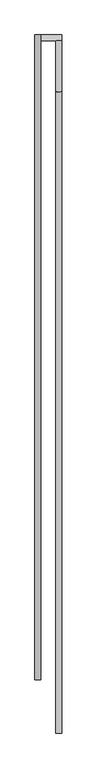
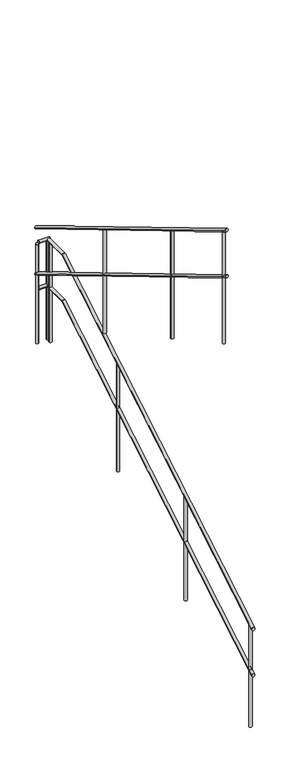
"""IFC4 building model written with IfcOpenShell, lengths in millimetres: railing geometry."""

from ifc_helpers import new_model, si_unit, point, frame, frame_2d, origin, place, context, project, spatial, circle_curve, ellipse_curve, trimmed, segment, composite_curve, outline, extrude, source, transform, mapped, element, save
from ifc_brep_helpers import plane_surface, cylinder_surface, advanced_brep


def railing_6fbbbaa8(model_context):
    return source(origin(), model_context, "Body", "SolidModel", [
        advanced_brep(
        [(11545.1052251, 14699.5208589, 749.8338893), (11515.1052251, 14699.5208589, 749.8338893), (11545.1052251, 18329.5208589, 2760.0), (11515.1052251, 18329.5208589, 2760.0), (11545.1052251, 18063.6609247, 2760.0), (11515.1052251, 18063.6609247, 2760.0)],
        [
            (0, 1, ellipse_curve(frame((11530.1052251, 14699.5208589, 749.8338893), z_axis=(0.0, -1.0, 0.0), x_axis=(0.0, 0.0, -1.0)), 17.4738031, 15.0)),
            (1, 0, ellipse_curve(frame((11530.1052251, 14699.5208589, 749.8338893), z_axis=(0.0, -1.0, 0.0), x_axis=(0.0, 0.0, -1.0)), 17.4738031, 15.0)),
            (2, 3, circle_curve(frame((11530.1052251, 18329.5208589, 2760.0), z_axis=(0.0, 1.0, 0.0), x_axis=(-1.0, 0.0, 0.0)), 15.0)),
            (3, 2, circle_curve(frame((11530.1052251, 18329.5208589, 2760.0), z_axis=(0.0, 1.0, 0.0), x_axis=(-1.0, 0.0, 0.0)), 15.0)),
            (0, 4),
            (4, 5, ellipse_curve(frame((11530.1052251, 18063.6609247, 2760.0), z_axis=(0.0, -0.9639574411334471, -0.26605648213012423), x_axis=(0.0, 0.2660564821301243, -0.9639574411334468)), 15.560853, 15.0)),
            (5, 1),
            (5, 4, ellipse_curve(frame((11530.1052251, 18063.6609247, 2760.0), z_axis=(0.0, -0.9639574411334471, -0.26605648213012423), x_axis=(0.0, 0.2660564821301243, -0.9639574411334468)), 15.560853, 15.0)),
            (4, 2),
            (3, 5),
        ],
        [
            plane_surface(frame((11530.1052251, 14699.5208589, 767.3076923), z_axis=(0.0, -1.0, 0.0), x_axis=(0.0, 0.0, 1.0))),
            plane_surface(frame((11530.1052251, 18329.5208589, 2775.0), z_axis=(0.0, 1.0, 0.0), x_axis=(0.0, 0.0, 1.0))),
            cylinder_surface(frame((11530.1052251, 14707.2148727, 754.4312739), z_axis=(0.0, -0.8584278966330859, -0.5129342514222422), x_axis=(-1.0, 0.0, 0.0)), 15.0),
            cylinder_surface(frame((11530.1052251, 18059.5208589, 2760.0), z_axis=(0.0, -1.0, 0.0), x_axis=(-1.0, 0.0, 0.0)), 15.0),
        ],
        [
            (0, [[1, 2]]),
            (1, [[3, 4]]),
            (2, [[-1, 5, 6, 7]]),
            (2, [[-2, -7, 8, -5]]),
            (3, [[-6, 9, -4, 10]]),
            (3, [[-8, -10, -3, -9]]),
        ],
    ),
        advanced_brep(
        [(11545.1052251, 18359.5208589, 2760.0), (11545.1052251, 18329.5208589, 2760.0), (11435.1052251, 18359.5208589, 2760.0), (11435.1052251, 18329.5208589, 2760.0)],
        [
            (0, 1, circle_curve(frame((11545.1052251, 18344.5208589, 2760.0), z_axis=(1.0, 0.0, 0.0), x_axis=(0.0, -1.0, 0.0)), 15.0)),
            (1, 0, circle_curve(frame((11545.1052251, 18344.5208589, 2760.0), z_axis=(1.0, 0.0, 0.0), x_axis=(0.0, -1.0, 0.0)), 15.0)),
            (2, 3, circle_curve(frame((11435.1052251, 18344.5208589, 2760.0), z_axis=(-1.0, 0.0, 0.0), x_axis=(0.0, -1.0, 0.0)), 15.0)),
            (3, 2, circle_curve(frame((11435.1052251, 18344.5208589, 2760.0), z_axis=(-1.0, 0.0, 0.0), x_axis=(0.0, -1.0, 0.0)), 15.0)),
            (0, 2),
            (3, 1),
        ],
        [
            plane_surface(frame((11545.1052251, 18344.5208589, 2775.0), z_axis=(1.0, 0.0, 0.0), x_axis=(0.0, -1.0, 0.0))),
            plane_surface(frame((11435.1052251, 18344.5208589, 2775.0), z_axis=(-1.0, 0.0, 0.0), x_axis=(0.0, -1.0, 0.0))),
            cylinder_surface(frame((11545.1052251, 18344.5208589, 2760.0), z_axis=(1.0, 0.0, 0.0), x_axis=(0.0, -1.0, 0.0)), 15.0),
        ],
        [
            (0, [[1, 2]]),
            (1, [[3, 4]]),
            (2, [[-1, 5, -4, 6]]),
            (2, [[-2, -6, -3, -5]]),
        ],
    ),
        advanced_brep(
        [(11405.1052251, 18359.5208589, 2912.8833398), (11435.1052251, 18359.5208589, 2912.8833398), (11405.1052251, 14979.5208589, 4932.5261969), (11435.1052251, 14979.5208589, 4932.5261969)],
        [
            (0, 1, ellipse_curve(frame((11420.1052251, 18359.5208589, 2912.8833398), z_axis=(0.0, 1.0, 0.0), x_axis=(0.0, 0.0, -1.0)), 17.4738031, 15.0)),
            (1, 0, ellipse_curve(frame((11420.1052251, 18359.5208589, 2912.8833398), z_axis=(0.0, 1.0, 0.0), x_axis=(0.0, 0.0, -1.0)), 17.4738031, 15.0)),
            (2, 3, ellipse_curve(frame((11420.1052251, 14979.5208589, 4932.5261969), z_axis=(0.0, -1.0, 0.0), x_axis=(0.0, 0.0, -1.0)), 17.4738031, 15.0)),
            (3, 2, ellipse_curve(frame((11420.1052251, 14979.5208589, 4932.5261969), z_axis=(0.0, -1.0, 0.0), x_axis=(0.0, 0.0, -1.0)), 17.4738031, 15.0)),
            (0, 2),
            (3, 1),
        ],
        [
            plane_surface(frame((11420.1052251, 18359.5208589, 2930.3571429), z_axis=(0.0, 1.0, 0.0), x_axis=(0.0, 0.0, -1.0))),
            plane_surface(frame((11420.1052251, 14979.5208589, 4950.0), z_axis=(0.0, -1.0, 0.0), x_axis=(0.0, 0.0, -1.0))),
            cylinder_surface(frame((11420.1052251, 18351.8268451, 2917.4807244), z_axis=(0.0, 0.8584278966330859, -0.5129342514222421), x_axis=(1.0, 0.0, 0.0)), 15.0),
        ],
        [
            (0, [[1, 2]]),
            (1, [[3, 4]]),
            (2, [[-1, 5, -4, 6]]),
            (2, [[-2, -6, -3, -5]]),
        ],
    ),
        advanced_brep(
        [(11545.1052251, 14699.5208589, 1249.8338893), (11515.1052251, 14699.5208589, 1249.8338893), (11545.1052251, 18063.6609247, 3260.0), (11515.1052251, 18063.6609247, 3260.0), (11545.1052251, 18329.5208589, 3260.0), (11515.1052251, 18329.5208589, 3260.0)],
        [
            (0, 1, ellipse_curve(frame((11530.1052251, 14699.5208589, 1249.8338893), z_axis=(0.0, -1.0, 0.0), x_axis=(0.0, 0.0, -1.0)), 17.4738031, 15.0)),
            (1, 0, ellipse_curve(frame((11530.1052251, 14699.5208589, 1249.8338893), z_axis=(0.0, -1.0, 0.0), x_axis=(0.0, 0.0, -1.0)), 17.4738031, 15.0)),
            (0, 2),
            (2, 3, ellipse_curve(frame((11530.1052251, 18063.6609247, 3260.0), z_axis=(0.0, -0.9639574411334471, -0.26605648213012423), x_axis=(0.0, 0.2660564821301243, -0.9639574411334468)), 15.560853, 15.0)),
            (3, 1),
            (3, 2, ellipse_curve(frame((11530.1052251, 18063.6609247, 3260.0), z_axis=(0.0, -0.9639574411334471, -0.26605648213012423), x_axis=(0.0, 0.2660564821301243, -0.9639574411334468)), 15.560853, 15.0)),
            (4, 5, circle_curve(frame((11530.1052251, 18329.5208589, 3260.0), z_axis=(0.0, 1.0, 0.0), x_axis=(-1.0, 0.0, 0.0)), 15.0)),
            (5, 4, circle_curve(frame((11530.1052251, 18329.5208589, 3260.0), z_axis=(0.0, 1.0, 0.0), x_axis=(-1.0, 0.0, 0.0)), 15.0)),
            (2, 4),
            (5, 3),
        ],
        [
            plane_surface(frame((11530.1052251, 14699.5208589, 1267.3076923), z_axis=(0.0, -1.0, 0.0), x_axis=(0.0, 0.0, 1.0))),
            cylinder_surface(frame((11530.1052251, 14707.2148727, 1254.4312739), z_axis=(0.0, -0.8584278966330859, -0.5129342514222422), x_axis=(-1.0, 0.0, 0.0)), 15.0),
            plane_surface(frame((11530.1052251, 18329.5208589, 3275.0), z_axis=(0.0, 1.0, 0.0), x_axis=(0.0, 0.0, 1.0))),
            cylinder_surface(frame((11530.1052251, 18059.5208589, 3260.0), z_axis=(0.0, -1.0, 0.0), x_axis=(-1.0, 0.0, 0.0)), 15.0),
        ],
        [
            (0, [[1, 2]]),
            (1, [[-1, 3, 4, 5]]),
            (1, [[-2, -5, 6, -3]]),
            (2, [[7, 8]]),
            (3, [[-4, 9, -8, 10]]),
            (3, [[-6, -10, -7, -9]]),
        ],
    ),
        advanced_brep(
        [(11545.1052251, 18359.5208589, 3260.0), (11545.1052251, 18329.5208589, 3260.0), (11435.1052251, 18359.5208589, 3260.0), (11435.1052251, 18329.5208589, 3260.0)],
        [
            (0, 1, circle_curve(frame((11545.1052251, 18344.5208589, 3260.0), z_axis=(1.0, 0.0, 0.0), x_axis=(0.0, -1.0, 0.0)), 15.0)),
            (1, 0, circle_curve(frame((11545.1052251, 18344.5208589, 3260.0), z_axis=(1.0, 0.0, 0.0), x_axis=(0.0, -1.0, 0.0)), 15.0)),
            (2, 3, circle_curve(frame((11435.1052251, 18344.5208589, 3260.0), z_axis=(-1.0, 0.0, 0.0), x_axis=(0.0, -1.0, 0.0)), 15.0)),
            (3, 2, circle_curve(frame((11435.1052251, 18344.5208589, 3260.0), z_axis=(-1.0, 0.0, 0.0), x_axis=(0.0, -1.0, 0.0)), 15.0)),
            (0, 2),
            (3, 1),
        ],
        [
            plane_surface(frame((11545.1052251, 18344.5208589, 3275.0), z_axis=(1.0, 0.0, 0.0), x_axis=(0.0, -1.0, 0.0))),
            plane_surface(frame((11435.1052251, 18344.5208589, 3275.0), z_axis=(-1.0, 0.0, 0.0), x_axis=(0.0, -1.0, 0.0))),
            cylinder_surface(frame((11545.1052251, 18344.5208589, 3260.0), z_axis=(1.0, 0.0, 0.0), x_axis=(0.0, -1.0, 0.0)), 15.0),
        ],
        [
            (0, [[1, 2]]),
            (1, [[3, 4]]),
            (2, [[-1, 5, -4, 6]]),
            (2, [[-2, -6, -3, -5]]),
        ],
    ),
        advanced_brep(
        [(11405.1052251, 18359.5208589, 3412.8833398), (11435.1052251, 18359.5208589, 3412.8833398), (11405.1052251, 14979.5208589, 5432.5261969), (11435.1052251, 14979.5208589, 5432.5261969)],
        [
            (0, 1, ellipse_curve(frame((11420.1052251, 18359.5208589, 3412.8833398), z_axis=(0.0, 1.0, 0.0), x_axis=(0.0, 0.0, -1.0)), 17.4738031, 15.0)),
            (1, 0, ellipse_curve(frame((11420.1052251, 18359.5208589, 3412.8833398), z_axis=(0.0, 1.0, 0.0), x_axis=(0.0, 0.0, -1.0)), 17.4738031, 15.0)),
            (2, 3, ellipse_curve(frame((11420.1052251, 14979.5208589, 5432.5261969), z_axis=(0.0, -1.0, 0.0), x_axis=(0.0, 0.0, -1.0)), 17.4738031, 15.0)),
            (3, 2, ellipse_curve(frame((11420.1052251, 14979.5208589, 5432.5261969), z_axis=(0.0, -1.0, 0.0), x_axis=(0.0, 0.0, -1.0)), 17.4738031, 15.0)),
            (0, 2),
            (3, 1),
        ],
        [
            plane_surface(frame((11420.1052251, 18359.5208589, 3430.3571429), z_axis=(0.0, 1.0, 0.0), x_axis=(0.0, 0.0, -1.0))),
            plane_surface(frame((11420.1052251, 14979.5208589, 5450.0), z_axis=(0.0, -1.0, 0.0), x_axis=(0.0, 0.0, -1.0))),
            cylinder_surface(frame((11420.1052251, 18351.8268451, 3417.4807244), z_axis=(0.0, 0.8584278966330859, -0.5129342514222421), x_axis=(1.0, 0.0, 0.0)), 15.0),
        ],
        [
            (0, [[1, 2]]),
            (1, [[3, 4]]),
            (2, [[-1, 5, -4, 6]]),
            (2, [[-2, -6, -3, -5]]),
        ],
    ),
        extrude(outline(composite_curve([segment(trimmed(circle_curve(frame_2d((11420.1052251, 15944.5208589)), 15.0), [point((11435.1052251, 15944.5208589))], [point((11405.1052251, 15944.5208589))], False, "CARTESIAN"), True, "CONTINUOUS"), segment(trimmed(circle_curve(frame_2d((11420.1052251, 15944.5208589)), 15.0), [point((11405.1052251, 15944.5208589))], [point((11435.1052251, 15944.5208589))], False, "CARTESIAN"), True, "CONTINUOUS")], self_intersect=False)), frame((0.0, 0.0, 3680.7692308), z_axis=(0.0, 0.0, 1.0), x_axis=(1.0, 0.0, 0.0)), (0.0, 0.0, 1.0), 1162.6167582),
        extrude(outline(composite_curve([segment(trimmed(circle_curve(frame_2d((11420.1052251, 17144.5208589)), 15.0), [point((11435.1052251, 17144.5208589))], [point((11405.1052251, 17144.5208589))], False, "CARTESIAN"), True, "CONTINUOUS"), segment(trimmed(circle_curve(frame_2d((11420.1052251, 17144.5208589)), 15.0), [point((11405.1052251, 17144.5208589))], [point((11435.1052251, 17144.5208589))], False, "CARTESIAN"), True, "CONTINUOUS")], self_intersect=False)), frame((0.0, 0.0, 3011.5384615), z_axis=(0.0, 0.0, 1.0), x_axis=(1.0, 0.0, 0.0)), (0.0, 0.0, 1.0), 1114.8145604),
        extrude(outline(composite_curve([segment(trimmed(circle_curve(frame_2d((11530.1052251, 18299.5208589)), 15.0), [point((11515.1052251, 18299.5208589))], [point((11545.1052251, 18299.5208589))], False, "CARTESIAN"), True, "CONTINUOUS"), segment(trimmed(circle_curve(frame_2d((11530.1052251, 18299.5208589)), 15.0), [point((11545.1052251, 18299.5208589))], [point((11515.1052251, 18299.5208589))], False, "CARTESIAN"), True, "CONTINUOUS")], self_intersect=False)), frame((0.0, 0.0, 2175.0), z_axis=(0.0, 0.0, 1.0), x_axis=(1.0, 0.0, 0.0)), (0.0, 0.0, 1.0), 1070.0),
        extrude(outline(composite_curve([segment(trimmed(circle_curve(frame_2d((11530.1052251, 17099.5208589)), 15.0), [point((11515.1052251, 17099.5208589))], [point((11545.1052251, 17099.5208589))], False, "CARTESIAN"), True, "CONTINUOUS"), segment(trimmed(circle_curve(frame_2d((11530.1052251, 17099.5208589)), 15.0), [point((11545.1052251, 17099.5208589))], [point((11515.1052251, 17099.5208589))], False, "CARTESIAN"), True, "CONTINUOUS")], self_intersect=False)), frame((0.0, 0.0, 1505.7692308), z_axis=(0.0, 0.0, 1.0), x_axis=(1.0, 0.0, 0.0)), (0.0, 0.0, 1.0), 1165.6043956),
        extrude(outline(composite_curve([segment(trimmed(circle_curve(frame_2d((11530.1052251, 15899.5208589)), 15.0), [point((11515.1052251, 15899.5208589))], [point((11545.1052251, 15899.5208589))], False, "CARTESIAN"), True, "CONTINUOUS"), segment(trimmed(circle_curve(frame_2d((11530.1052251, 15899.5208589)), 15.0), [point((11545.1052251, 15899.5208589))], [point((11515.1052251, 15899.5208589))], False, "CARTESIAN"), True, "CONTINUOUS")], self_intersect=False)), frame((0.0, 0.0, 836.5384615), z_axis=(0.0, 0.0, 1.0), x_axis=(1.0, 0.0, 0.0)), (0.0, 0.0, 1.0), 1117.8021978),
        extrude(outline(composite_curve([segment(trimmed(circle_curve(frame_2d((11420.1052251, 18344.5208589)), 15.0), [point((11420.1052251, 18329.5208589))], [point((11420.1052251, 18359.5208589))], False, "CARTESIAN"), True, "CONTINUOUS"), segment(trimmed(circle_curve(frame_2d((11420.1052251, 18344.5208589)), 15.0), [point((11420.1052251, 18359.5208589))], [point((11420.1052251, 18329.5208589))], False, "CARTESIAN"), True, "CONTINUOUS")], self_intersect=False)), frame((0.0, 0.0, 2175.0), z_axis=(0.0, 0.0, 1.0), x_axis=(1.0, 0.0, 0.0)), (0.0, 0.0, 1.0), 1070.0),
        extrude(outline(composite_curve([segment(trimmed(circle_curve(frame_2d((11530.1052251, 18344.5208589)), 15.0), [point((11515.1052251, 18344.5208589))], [point((11545.1052251, 18344.5208589))], False, "CARTESIAN"), True, "CONTINUOUS"), segment(trimmed(circle_curve(frame_2d((11530.1052251, 18344.5208589)), 15.0), [point((11545.1052251, 18344.5208589))], [point((11515.1052251, 18344.5208589))], False, "CARTESIAN"), True, "CONTINUOUS")], self_intersect=False)), frame((0.0, 0.0, 2175.0), z_axis=(0.0, 0.0, 1.0), x_axis=(1.0, 0.0, 0.0)), (0.0, 0.0, 1.0), 1070.0),
        extrude(outline(composite_curve([segment(trimmed(circle_curve(frame_2d((11420.1052251, 15029.5208589)), 15.0), [point((11435.1052251, 15029.5208589))], [point((11405.1052251, 15029.5208589))], False, "CARTESIAN"), True, "CONTINUOUS"), segment(trimmed(circle_curve(frame_2d((11420.1052251, 15029.5208589)), 15.0), [point((11405.1052251, 15029.5208589))], [point((11435.1052251, 15029.5208589))], False, "CARTESIAN"), True, "CONTINUOUS")], self_intersect=False)), frame((0.0, 0.0, 4182.6923077), z_axis=(0.0, 0.0, 1.0), x_axis=(1.0, 0.0, 0.0)), (0.0, 0.0, 1.0), 1207.4313187),
        extrude(outline(composite_curve([segment(trimmed(circle_curve(frame_2d((11530.1052251, 14749.5208589)), 15.0), [point((11515.1052251, 14749.5208589))], [point((11545.1052251, 14749.5208589))], False, "CARTESIAN"), True, "CONTINUOUS"), segment(trimmed(circle_curve(frame_2d((11530.1052251, 14749.5208589)), 15.0), [point((11545.1052251, 14749.5208589))], [point((11515.1052251, 14749.5208589))], False, "CARTESIAN"), True, "CONTINUOUS")], self_intersect=False)), frame((0.0, 0.0, 167.3076923), z_axis=(0.0, 0.0, 1.0), x_axis=(1.0, 0.0, 0.0)), (0.0, 0.0, 1.0), 1099.8763736),
    ])


if __name__ == "__main__":
    model = new_model("IFC4")
    model_context = context("Model", 3, world=origin())
    ifc_project = project(units=[si_unit("LENGTHUNIT", "METRE", prefix="MILLI")], contexts=[model_context])
    site = spatial("IfcSite", under=ifc_project)
    building = spatial("IfcBuilding", under=site)
    placement = place(None, origin())
    railing_shape = railing_6fbbbaa8(model_context)
    element("IfcRailing", 1, at=placement, inside=building, context=model_context, shape_type="MappedRepresentation", body=[
        mapped(railing_shape, transform((0.0, 0.0, 0.0), x_axis=(1.0, 0.0, 0.0), y_axis=(0.0, 1.0, 0.0), z_axis=(0.0, 0.0, 1.0))),
    ])
    save(model, "model.ifc")
